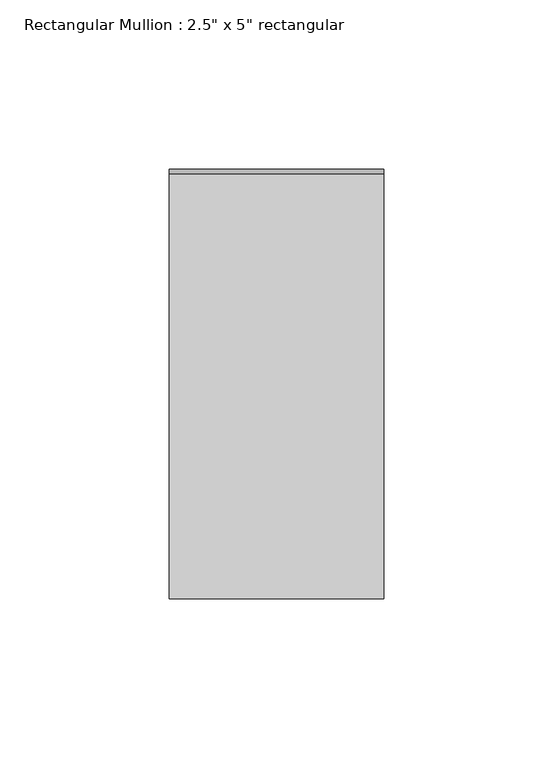
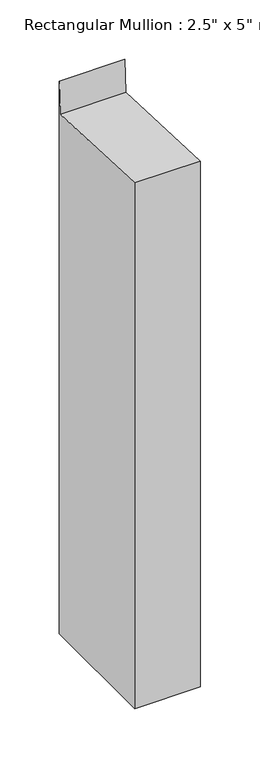
"""IFC4 building model written with IfcOpenShell, lengths in millimetres: member geometry."""

from ifc_helpers import new_model, si_unit, frame, origin, place, context, project, spatial, polyline, outline, extrude, source, transform, mapped, element, save


def member_24c26854(model_context):
    return source(origin(), model_context, "Body", "SweptSolid", [
        extrude(outline(polyline([(-63.5, 2.6913332), (62.0828234, -2.6888667), (63.5, 30.390395), (63.5, -537.627929), (-63.5, -537.627929), (-63.5, 2.6913332)])), frame((-63.5, 0.0, 0.0), z_axis=(1.0, 0.0, 0.0), x_axis=(0.0, 1.0, 0.0)), (0.0, 0.0, 1.0), 63.5),
    ])


if __name__ == "__main__":
    model = new_model("IFC4")
    model_context = context("Model", 3, world=origin())
    ifc_project = project(units=[si_unit("LENGTHUNIT", "METRE", prefix="MILLI")], contexts=[model_context])
    site = spatial("IfcSite", under=ifc_project)
    building = spatial("IfcBuilding", under=site)
    placement = place(None, origin())
    member_shape = member_24c26854(model_context)
    element("IfcMember", 1, ObjectType="Rectangular Mullion : 2.5\" x 5\" rectangular", at=placement, inside=building, context=model_context, shape_type="MappedRepresentation", body=[
        mapped(member_shape, transform((0.0, 0.0, 0.0), x_axis=(1.0, 0.0, 0.0), y_axis=(0.0, 1.0, 0.0), z_axis=(0.0, 0.0, 1.0))),
    ])
    save(model, "model.ifc")

# Revit data of these elements
# Type "Rectangular Mullion : 2.5\" x 5\" rectangular"
#   built-in parameter 1007304 = 0.416667 (stored number, unit not read)
#   built-in parameter 1007301 = 0.104167 (stored number, unit not read)
#   built-in parameter 1007300 = 0.104167 (stored number, unit not read)
# Element 1 (IfcMember, "Rectangular Mullion : 2.5\" x 5\" rectangular")
#   Materials on its faces: "Metal - Aluminum"
# Materials
#   "Metal - Aluminum": class "Metal", colour RGB 247 247 247, transparency 0, Cost = 0
